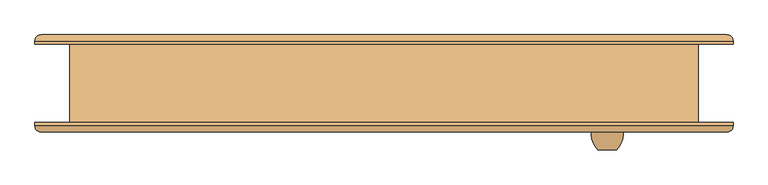
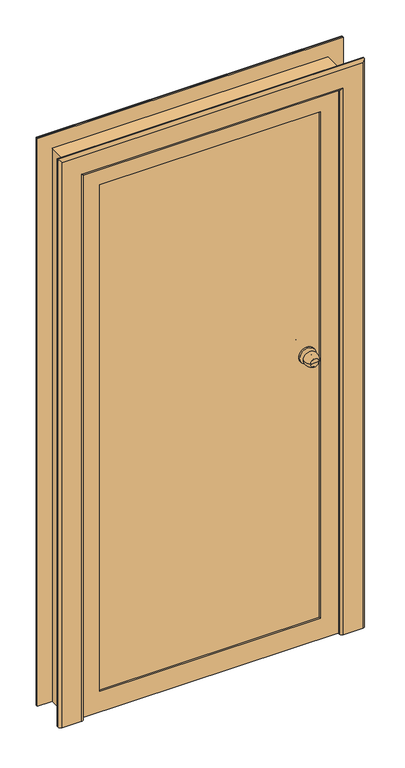
"""IFC4 building model written with IfcOpenShell, lengths in millimetres: door geometry, Наружная дверь 1-Навесная - Один проем наружу с порогом - 31173-2003 : ДСН КЛН  М1 УЗ 2100-1000 ГОСТ 31173-2003 2."""

from ifc_helpers import new_model, si_unit, point, frame, origin, place, context, project, spatial, polyline, circle_curve, ellipse_curve, trimmed, outline, extrude, faceted_brep, source, transform, mapped, element, save
from ifc_brep_helpers import plane_surface, cylinder_surface, revolved_surface, advanced_brep


def door_ae19c2ee(model_context):
    return source(origin(), model_context, "Body", "SolidModel", [
        advanced_brep(
        [(340.0, -105.5, 1100.0), (355.0, -105.5, 1100.0), (370.0, -105.5, 1100.0), (380.0, -75.5, 1100.0), (330.0, -75.5, 1100.0), (373.0, -75.5, 1100.0), (337.0, -75.5, 1100.0), (365.0, -67.5, 1100.0), (345.0, -67.5, 1100.0), (365.0, -61.5, 1100.0), (345.0, -61.5, 1100.0), (385.0, -61.5, 1100.0), (325.0, -61.5, 1100.0), (385.0, -55.5, 1100.0), (325.0, -55.5, 1100.0)],
        [
            (0, 1),
            (1, 2),
            (2, 0, circle_curve(frame((355.0, -105.5, 1100.0), z_axis=(0.0, -1.0, 0.0), x_axis=(1.0, 0.0, 0.0)), 15.0)),
            (0, 2, circle_curve(frame((355.0, -105.5, 1100.0), z_axis=(0.0, -1.0, 0.0), x_axis=(1.0, 0.0, 0.0)), 15.0)),
            (2, 3, circle_curve(frame((345.3773735, -80.6257912, 1100.0), z_axis=(0.0, 0.0, 1.0), x_axis=(-1.0, 0.0, 0.0)), 35.0)),
            (3, 4, circle_curve(frame((355.0, -75.5, 1100.0), z_axis=(0.0, -1.0, 0.0), x_axis=(1.0, 0.0, 0.0)), 25.0)),
            (4, 0, circle_curve(frame((364.6226265, -80.6257912, 1100.0), z_axis=(0.0, 0.0, 1.0), x_axis=(1.0, 0.0, 0.0)), 35.0)),
            (4, 3, circle_curve(frame((355.0, -75.5, 1100.0), z_axis=(0.0, -1.0, 0.0), x_axis=(1.0, 0.0, 0.0)), 25.0)),
            (3, 5),
            (5, 6, circle_curve(frame((355.0, -75.5, 1100.0), z_axis=(0.0, -1.0, 0.0), x_axis=(1.0, 0.0, 0.0)), 18.0)),
            (6, 4),
            (6, 5, circle_curve(frame((355.0, -75.5, 1100.0), z_axis=(0.0, -1.0, 0.0), x_axis=(1.0, 0.0, 0.0)), 18.0)),
            (5, 7, circle_curve(frame((373.0, -67.5, 1100.0), z_axis=(0.0, 0.0, -1.0), x_axis=(-1.0, 0.0, 0.0)), 8.0)),
            (7, 8, circle_curve(frame((355.0, -67.5, 1100.0), z_axis=(0.0, -1.0, 0.0), x_axis=(1.0, 0.0, 0.0)), 10.0)),
            (8, 6, circle_curve(frame((337.0, -67.5, 1100.0), z_axis=(0.0, 0.0, -1.0), x_axis=(1.0, 0.0, 0.0)), 8.0)),
            (8, 7, circle_curve(frame((355.0, -67.5, 1100.0), z_axis=(0.0, -1.0, 0.0), x_axis=(1.0, 0.0, 0.0)), 10.0)),
            (7, 9),
            (9, 10, circle_curve(frame((355.0, -61.5, 1100.0), z_axis=(0.0, -1.0, 0.0), x_axis=(1.0, 0.0, 0.0)), 10.0)),
            (10, 8),
            (10, 9, circle_curve(frame((355.0, -61.5, 1100.0), z_axis=(0.0, -1.0, 0.0), x_axis=(1.0, 0.0, 0.0)), 10.0)),
            (11, 12, circle_curve(frame((355.0, -61.5, 1100.0), z_axis=(0.0, -1.0, 0.0), x_axis=(-1.0, 0.0, 0.0)), 30.0)),
            (12, 11, circle_curve(frame((355.0, -61.5, 1100.0), z_axis=(0.0, -1.0, 0.0), x_axis=(-1.0, 0.0, 0.0)), 30.0)),
            (13, 14, circle_curve(frame((355.0, -55.5, 1100.0), z_axis=(0.0, 1.0, 0.0), x_axis=(-1.0, 0.0, 0.0)), 30.0)),
            (14, 13, circle_curve(frame((355.0, -55.5, 1100.0), z_axis=(0.0, 1.0, 0.0), x_axis=(-1.0, 0.0, 0.0)), 30.0)),
            (12, 14),
            (13, 11),
        ],
        [
            plane_surface(frame((355.0, -105.5, 1100.0), z_axis=(0.0, -1.0, 0.0), x_axis=(1.0, 0.0, 0.0))),
            revolved_surface(trimmed(ellipse_curve(frame((345.3773735, -80.6257912, 1100.0), z_axis=(0.0, 0.0, 1.0), x_axis=(-1.0, 0.0, 0.0)), 35.0, 35.0), [point((370.0, -105.5, 1100.0))], [point((380.0, -75.5, 1100.0))], True, "CARTESIAN"), (355.0, -135.5, 1100.0), (0.0, 1.0, 0.0)),
            plane_surface(frame((355.0, -75.5, 1100.0), z_axis=(0.0, 1.0, 0.0), x_axis=(1.0, 0.0, 0.0))),
            revolved_surface(trimmed(ellipse_curve(frame((373.0, -67.5, 1100.0), z_axis=(0.0, 0.0, -1.0), x_axis=(-1.0, 0.0, 0.0)), 8.0, 8.0), [point((373.0, -75.5, 1100.0))], [point((365.0, -67.5, 1100.0))], True, "CARTESIAN"), (355.0, -135.5, 1100.0), (0.0, 1.0, 0.0)),
            cylinder_surface(frame((355.0, -135.5, 1100.0), z_axis=(0.0, 1.0, 0.0), x_axis=(1.0, 0.0, 0.0)), 10.0),
            plane_surface(frame((325.0, -61.5, 1100.0), z_axis=(0.0, -1.0, 0.0), x_axis=(0.0, 0.0, 1.0))),
            plane_surface(frame((325.0, -55.5, 1100.0), z_axis=(0.0, 1.0, 0.0), x_axis=(0.0, 0.0, -1.0))),
            cylinder_surface(frame((355.0, -55.5, 1100.0), z_axis=(0.0, -1.0, 0.0), x_axis=(-1.0, 0.0, 0.0)), 30.0),
        ],
        [
            (0, [[1, 2, 3]]),
            (0, [[-1, 4, -2]]),
            (1, [[5, 6, 7, -3]]),
            (1, [[-7, 8, -5, -4]]),
            (2, [[9, 10, 11, -6]]),
            (2, [[-11, 12, -9, -8]]),
            (3, [[13, 14, 15, -10]]),
            (3, [[-15, 16, -13, -12]]),
            (4, [[17, 18, 19, -14]]),
            (4, [[-19, 20, -17, -16]]),
            (5, [[21, 22], [-20, -18]]),
            (6, [[23, 24]]),
            (7, [[25, -23, 26, -22]]),
            (7, [[-26, -24, -25, -21]]),
        ],
    ),
        advanced_brep(
        [(370.0, 64.5, 1100.0), (355.0, 64.5, 1100.0), (340.0, 64.5, 1100.0), (330.0, 34.5, 1100.0), (380.0, 34.5, 1100.0), (337.0, 34.5, 1100.0), (373.0, 34.5, 1100.0), (345.0, 26.5, 1100.0), (365.0, 26.5, 1100.0), (345.0, 20.5, 1100.0), (365.0, 20.5, 1100.0), (325.0, 20.5, 1100.0), (385.0, 20.5, 1100.0), (325.0, 14.5, 1100.0), (385.0, 14.5, 1100.0)],
        [
            (0, 1),
            (1, 2),
            (2, 0, circle_curve(frame((355.0, 64.5, 1100.0), z_axis=(0.0, 1.0, 0.0), x_axis=(-1.0, 0.0, 0.0)), 15.0)),
            (0, 2, circle_curve(frame((355.0, 64.5, 1100.0), z_axis=(0.0, 1.0, 0.0), x_axis=(-1.0, 0.0, 0.0)), 15.0)),
            (2, 3, circle_curve(frame((364.6226265, 39.6257912, 1100.0), z_axis=(0.0, 0.0, 1.0), x_axis=(1.0, 0.0, 0.0)), 35.0)),
            (3, 4, circle_curve(frame((355.0, 34.5, 1100.0), z_axis=(0.0, 1.0, 0.0), x_axis=(-1.0, 0.0, 0.0)), 25.0)),
            (4, 0, circle_curve(frame((345.3773735, 39.6257912, 1100.0), z_axis=(0.0, 0.0, 1.0), x_axis=(-1.0, 0.0, 0.0)), 35.0)),
            (4, 3, circle_curve(frame((355.0, 34.5, 1100.0), z_axis=(0.0, 1.0, 0.0), x_axis=(-1.0, 0.0, 0.0)), 25.0)),
            (3, 5),
            (5, 6, circle_curve(frame((355.0, 34.5, 1100.0), z_axis=(0.0, 1.0, 0.0), x_axis=(-1.0, 0.0, 0.0)), 18.0)),
            (6, 4),
            (6, 5, circle_curve(frame((355.0, 34.5, 1100.0), z_axis=(0.0, 1.0, 0.0), x_axis=(-1.0, 0.0, 0.0)), 18.0)),
            (5, 7, circle_curve(frame((337.0, 26.5, 1100.0), z_axis=(0.0, 0.0, -1.0), x_axis=(1.0, 0.0, 0.0)), 8.0)),
            (7, 8, circle_curve(frame((355.0, 26.5, 1100.0), z_axis=(0.0, 1.0, 0.0), x_axis=(-1.0, 0.0, 0.0)), 10.0)),
            (8, 6, circle_curve(frame((373.0, 26.5, 1100.0), z_axis=(0.0, 0.0, -1.0), x_axis=(-1.0, 0.0, 0.0)), 8.0)),
            (8, 7, circle_curve(frame((355.0, 26.5, 1100.0), z_axis=(0.0, 1.0, 0.0), x_axis=(-1.0, 0.0, 0.0)), 10.0)),
            (7, 9),
            (9, 10, circle_curve(frame((355.0, 20.5, 1100.0), z_axis=(0.0, 1.0, 0.0), x_axis=(-1.0, 0.0, 0.0)), 10.0)),
            (10, 8),
            (10, 9, circle_curve(frame((355.0, 20.5, 1100.0), z_axis=(0.0, 1.0, 0.0), x_axis=(-1.0, 0.0, 0.0)), 10.0)),
            (11, 12, circle_curve(frame((355.0, 20.5, 1100.0), z_axis=(0.0, 1.0, 0.0), x_axis=(1.0, 0.0, 0.0)), 30.0)),
            (12, 11, circle_curve(frame((355.0, 20.5, 1100.0), z_axis=(0.0, 1.0, 0.0), x_axis=(1.0, 0.0, 0.0)), 30.0)),
            (13, 14, circle_curve(frame((355.0, 14.5, 1100.0), z_axis=(0.0, -1.0, 0.0), x_axis=(1.0, 0.0, 0.0)), 30.0)),
            (14, 13, circle_curve(frame((355.0, 14.5, 1100.0), z_axis=(0.0, -1.0, 0.0), x_axis=(1.0, 0.0, 0.0)), 30.0)),
            (12, 14),
            (13, 11),
        ],
        [
            plane_surface(frame((355.0, 64.5, 1100.0), z_axis=(0.0, 1.0, 0.0), x_axis=(-1.0, 0.0, 0.0))),
            revolved_surface(trimmed(ellipse_curve(frame((364.6226265, 39.6257912, 1100.0), z_axis=(0.0, 0.0, 1.0), x_axis=(1.0, 0.0, 0.0)), 35.0, 35.0), [point((340.0, 64.5, 1100.0))], [point((330.0, 34.5, 1100.0))], True, "CARTESIAN"), (355.0, 94.5, 1100.0), (0.0, -1.0, 0.0)),
            plane_surface(frame((355.0, 34.5, 1100.0), z_axis=(0.0, -1.0, 0.0), x_axis=(-1.0, 0.0, 0.0))),
            revolved_surface(trimmed(ellipse_curve(frame((337.0, 26.5, 1100.0), z_axis=(0.0, 0.0, -1.0), x_axis=(1.0, 0.0, 0.0)), 8.0, 8.0), [point((337.0, 34.5, 1100.0))], [point((345.0, 26.5, 1100.0))], True, "CARTESIAN"), (355.0, 94.5, 1100.0), (0.0, -1.0, 0.0)),
            cylinder_surface(frame((355.0, 94.5, 1100.0), z_axis=(0.0, -1.0, 0.0), x_axis=(-1.0, 0.0, 0.0)), 10.0),
            plane_surface(frame((385.0, 20.5, 1100.0), z_axis=(0.0, 1.0, 0.0), x_axis=(0.0, 0.0, 1.0))),
            plane_surface(frame((385.0, 14.5, 1100.0), z_axis=(0.0, -1.0, 0.0), x_axis=(0.0, 0.0, -1.0))),
            cylinder_surface(frame((355.0, 14.5, 1100.0), z_axis=(0.0, 1.0, 0.0), x_axis=(1.0, 0.0, 0.0)), 30.0),
        ],
        [
            (0, [[1, 2, 3]]),
            (0, [[-1, 4, -2]]),
            (1, [[5, 6, 7, -3]]),
            (1, [[-7, 8, -5, -4]]),
            (2, [[9, 10, 11, -6]]),
            (2, [[-11, 12, -9, -8]]),
            (3, [[13, 14, 15, -10]]),
            (3, [[-15, 16, -13, -12]]),
            (4, [[17, 18, 19, -14]]),
            (4, [[-19, 20, -17, -16]]),
            (5, [[21, 22], [-20, -18]]),
            (6, [[23, 24]]),
            (7, [[25, -23, 26, -22]]),
            (7, [[-26, -24, -25, -21]]),
        ],
    ),
        faceted_brep([(435.0, 14.5, 42.0), (435.0, 9.5, 42.0), (-435.0, 9.5, 42.0), (-435.0, 14.5, 42.0), (435.0, 14.5, 2055.0), (435.0, 9.5, 2055.0), (-435.0, 9.5, 2055.0), (415.0, 9.5, 2035.0), (415.0, 9.5, 62.0), (-415.0, 9.5, 62.0), (-415.0, 9.5, 2035.0), (-435.0, 14.5, 2055.0), (415.0, -55.5, 2035.0), (415.0, -55.5, 62.0), (-415.0, -55.5, 62.0), (-415.0, -55.5, 2035.0)], [[[0, 1, 2, 3]], [[4, 5, 1, 0]], [[5, 6, 2, 1], [7, 8, 9, 10]], [[2, 6, 11, 3]], [[11, 4, 0, 3]], [[7, 12, 13, 8]], [[9, 8, 13, 14]], [[15, 10, 9, 14]], [[12, 15, 14, 13]], [[4, 11, 6, 5]], [[7, 10, 15, 12]]]),
        extrude(outline(polyline([(0.0, 465.0), (0.0, 480.0), (2100.0, 480.0), (2100.0, -480.0), (0.0, -480.0), (0.0, -465.0), (2085.0, -465.0), (2085.0, 465.0), (0.0, 465.0)])), frame((0.0, 7.5, 0.0), z_axis=(0.0, 1.0, 0.0), x_axis=(0.0, 0.0, 1.0)), (0.0, 0.0, 1.0), 55.0),
        faceted_brep([(480.0, 7.5, 0.0), (480.0, -62.5, 0.0), (-480.0, -62.5, 0.0), (-480.0, 7.5, 0.0), (-480.0, -62.5, 2100.0), (-480.0, 7.5, 2100.0), (480.0, -62.5, 2100.0), (-400.0, -62.5, 2020.0), (400.0, -62.5, 2020.0), (400.0, -62.5, 80.0), (-400.0, -62.5, 80.0), (480.0, 7.5, 2100.0), (-420.0, 7.5, 60.0), (420.0, 7.5, 60.0), (420.0, 7.5, 2040.0), (-420.0, 7.5, 2040.0), (420.0, -57.5, 60.0), (-420.0, -57.5, 60.0), (-420.0, -57.5, 2040.0), (420.0, -57.5, 2040.0), (-400.0, -57.5, 80.0), (400.0, -57.5, 80.0), (400.0, -57.5, 2020.0), (-400.0, -57.5, 2020.0)], [[[0, 1, 2, 3]], [[3, 2, 4, 5]], [[2, 1, 6, 4], [7, 8, 9, 10]], [[5, 11, 0, 3], [12, 13, 14, 15]], [[16, 13, 12, 17]], [[17, 12, 15, 18]], [[18, 19, 16, 17], [20, 21, 22, 23]], [[9, 21, 20, 10]], [[10, 20, 23, 7]], [[11, 6, 1, 0]], [[19, 14, 13, 16]], [[8, 22, 21, 9]], [[5, 4, 6, 11]], [[18, 15, 14, 19]], [[7, 23, 22, 8]]]),
        advanced_brep(
        [(-555.0, -62.5, 0.0), (-465.0, -62.5, 0.0), (-465.0, -67.5, 0.0), (-475.0, -77.5, 0.0), (-545.0, -77.5, 0.0), (-555.0, -67.5, 0.0), (-555.0, -62.5, 2175.0), (555.0, -62.5, 2175.0), (555.0, -62.5, 0.0), (465.0, -62.5, 0.0), (465.0, -62.5, 2085.0), (-465.0, -62.5, 2085.0), (-465.0, -67.5, 2085.0), (-475.0, -77.5, 2095.0), (475.0, -77.5, 2095.0), (475.0, -77.5, 0.0), (545.0, -77.5, 0.0), (545.0, -77.5, 2165.0), (-545.0, -77.5, 2165.0), (-555.0, -67.5, 2175.0), (555.0, -67.5, 2175.0), (555.0, -67.5, 0.0), (465.0, -67.5, 0.0), (465.0, -67.5, 2085.0)],
        [
            (0, 1),
            (1, 2),
            (2, 3, circle_curve(frame((-475.0, -67.5, 0.0), z_axis=(0.0, 0.0, -1.0), x_axis=(-1.0, 0.0, 0.0)), 10.0)),
            (3, 4),
            (4, 5, circle_curve(frame((-545.0, -67.5, 0.0), z_axis=(0.0, 0.0, -1.0), x_axis=(-1.0, 0.0, 0.0)), 10.0)),
            (5, 0),
            (0, 6),
            (6, 7),
            (7, 8),
            (8, 9),
            (9, 10),
            (10, 11),
            (11, 1),
            (11, 12),
            (12, 2),
            (12, 13, ellipse_curve(frame((-475.0, -67.5, 2095.0), z_axis=(-0.7071067811865475, 0.0, -0.7071067811865475), x_axis=(0.7071067811865474, 0.0, -0.7071067811865476)), 14.1421356, 10.0)),
            (13, 3),
            (13, 14),
            (14, 15),
            (15, 16),
            (16, 17),
            (17, 18),
            (18, 4),
            (18, 19, ellipse_curve(frame((-545.0, -67.5, 2165.0), z_axis=(-0.7071067811865475, 0.0, -0.7071067811865475), x_axis=(0.7071067811865474, 0.0, -0.7071067811865476)), 14.1421356, 10.0)),
            (19, 5),
            (19, 6),
            (7, 20),
            (20, 21),
            (21, 8),
            (21, 16, circle_curve(frame((545.0, -67.5, 0.0), z_axis=(0.0, 0.0, -1.0), x_axis=(1.0, 0.0, 0.0)), 10.0)),
            (15, 22, circle_curve(frame((475.0, -67.5, 0.0), z_axis=(0.0, 0.0, -1.0), x_axis=(1.0, 0.0, 0.0)), 10.0)),
            (22, 9),
            (23, 10),
            (22, 23),
            (14, 23, ellipse_curve(frame((475.0, -67.5, 2095.0), z_axis=(0.7071067811865475, 0.0, -0.7071067811865475), x_axis=(0.7071067811865474, 0.0, 0.7071067811865476)), 14.1421356, 10.0)),
            (20, 17, ellipse_curve(frame((545.0, -67.5, 2165.0), z_axis=(0.7071067811865475, 0.0, -0.7071067811865475), x_axis=(0.7071067811865474, 0.0, 0.7071067811865476)), 14.1421356, 10.0)),
            (23, 12),
            (20, 19),
        ],
        [
            plane_surface(frame((-500.0, -62.5, 0.0), z_axis=(0.0, 0.0, -1.0), x_axis=(0.0, -1.0, 0.0))),
            plane_surface(frame((-555.0, -62.5, 0.0), z_axis=(0.0, 1.0, 0.0), x_axis=(0.0, 0.0, 1.0))),
            plane_surface(frame((-465.0, -62.5, 0.0), z_axis=(1.0, 0.0, 0.0), x_axis=(0.0, 0.0, 1.0))),
            cylinder_surface(frame((-475.0, -67.5, 0.0), z_axis=(0.0, 0.0, -1.0), x_axis=(-1.0, 0.0, 0.0)), 10.0),
            plane_surface(frame((-475.0, -77.5, 0.0), z_axis=(0.0, -1.0, 0.0), x_axis=(0.0, 0.0, 1.0))),
            cylinder_surface(frame((-545.0, -67.5, 0.0), z_axis=(0.0, 0.0, -1.0), x_axis=(-1.0, 0.0, 0.0)), 10.0),
            plane_surface(frame((-555.0, -67.5, 0.0), z_axis=(-1.0, 0.0, 0.0), x_axis=(0.0, 0.0, 1.0))),
            plane_surface(frame((555.0, -67.5, 2175.0), z_axis=(1.0, 0.0, 0.0), x_axis=(0.0, 0.0, -1.0))),
            plane_surface(frame((500.0, -62.5, 0.0), z_axis=(0.0, 0.0, -1.0), x_axis=(0.0, -1.0, 0.0))),
            plane_surface(frame((465.0, -62.5, 2085.0), z_axis=(-1.0, 0.0, 0.0), x_axis=(0.0, 0.0, -1.0))),
            cylinder_surface(frame((475.0, -67.5, 2120.0), z_axis=(0.0, 0.0, 1.0), x_axis=(1.0, 0.0, 0.0)), 10.0),
            cylinder_surface(frame((545.0, -67.5, 2120.0), z_axis=(0.0, 0.0, 1.0), x_axis=(1.0, 0.0, 0.0)), 10.0),
            plane_surface(frame((-465.0, -62.5, 2085.0), z_axis=(0.0, 0.0, -1.0), x_axis=(1.0, 0.0, 0.0))),
            cylinder_surface(frame((-500.0, -67.5, 2095.0), z_axis=(-1.0, 0.0, 0.0), x_axis=(0.0, 0.0, 1.0)), 10.0),
            cylinder_surface(frame((-500.0, -67.5, 2165.0), z_axis=(-1.0, 0.0, 0.0), x_axis=(0.0, 0.0, 1.0)), 10.0),
            plane_surface(frame((-555.0, -67.5, 2175.0), z_axis=(0.0, 0.0, 1.0), x_axis=(1.0, 0.0, 0.0))),
        ],
        [
            (0, [[1, 2, 3, 4, 5, 6]]),
            (1, [[-1, 7, 8, 9, 10, 11, 12, 13]]),
            (2, [[-2, -13, 14, 15]]),
            (3, [[-3, -15, 16, 17]]),
            (4, [[-4, -17, 18, 19, 20, 21, 22, 23]]),
            (5, [[-5, -23, 24, 25]]),
            (6, [[-6, -25, 26, -7]]),
            (7, [[27, 28, 29, -9]]),
            (8, [[-29, 30, -20, 31, 32, -10]]),
            (9, [[33, -11, -32, 34]]),
            (10, [[35, -34, -31, -19]]),
            (11, [[36, -21, -30, -28]]),
            (12, [[-14, -12, -33, 37]]),
            (13, [[-16, -37, -35, -18]]),
            (14, [[-24, -22, -36, 38]]),
            (15, [[-26, -38, -27, -8]]),
        ],
    ),
        advanced_brep(
        [(555.0, 62.5, 0.0), (465.0, 62.5, 0.0), (465.0, 67.5, 0.0), (475.0, 77.5, 0.0), (545.0, 77.5, 0.0), (555.0, 67.5, 0.0), (555.0, 62.5, 2175.0), (-555.0, 62.5, 2175.0), (-555.0, 62.5, 0.0), (-465.0, 62.5, 0.0), (-465.0, 62.5, 2085.0), (465.0, 62.5, 2085.0), (465.0, 67.5, 2085.0), (475.0, 77.5, 2095.0), (-475.0, 77.5, 2095.0), (-475.0, 77.5, 0.0), (-545.0, 77.5, 0.0), (-545.0, 77.5, 2165.0), (545.0, 77.5, 2165.0), (555.0, 67.5, 2175.0), (-555.0, 67.5, 2175.0), (-555.0, 67.5, 0.0), (-465.0, 67.5, 0.0), (-465.0, 67.5, 2085.0)],
        [
            (0, 1),
            (1, 2),
            (2, 3, circle_curve(frame((475.0, 67.5, 0.0), z_axis=(0.0, 0.0, -1.0), x_axis=(1.0, 0.0, 0.0)), 10.0)),
            (3, 4),
            (4, 5, circle_curve(frame((545.0, 67.5, 0.0), z_axis=(0.0, 0.0, -1.0), x_axis=(1.0, 0.0, 0.0)), 10.0)),
            (5, 0),
            (0, 6),
            (6, 7),
            (7, 8),
            (8, 9),
            (9, 10),
            (10, 11),
            (11, 1),
            (11, 12),
            (12, 2),
            (12, 13, ellipse_curve(frame((475.0, 67.5, 2095.0), z_axis=(0.7071067811865475, 0.0, -0.7071067811865475), x_axis=(-0.7071067811865474, 0.0, -0.7071067811865476)), 14.1421356, 10.0)),
            (13, 3),
            (13, 14),
            (14, 15),
            (15, 16),
            (16, 17),
            (17, 18),
            (18, 4),
            (18, 19, ellipse_curve(frame((545.0, 67.5, 2165.0), z_axis=(0.7071067811865475, 0.0, -0.7071067811865475), x_axis=(-0.7071067811865474, 0.0, -0.7071067811865476)), 14.1421356, 10.0)),
            (19, 5),
            (19, 6),
            (7, 20),
            (20, 21),
            (21, 8),
            (21, 16, circle_curve(frame((-545.0, 67.5, 0.0), z_axis=(0.0, 0.0, -1.0), x_axis=(-1.0, 0.0, 0.0)), 10.0)),
            (15, 22, circle_curve(frame((-475.0, 67.5, 0.0), z_axis=(0.0, 0.0, -1.0), x_axis=(-1.0, 0.0, 0.0)), 10.0)),
            (22, 9),
            (23, 10),
            (22, 23),
            (14, 23, ellipse_curve(frame((-475.0, 67.5, 2095.0), z_axis=(-0.7071067811865475, 0.0, -0.7071067811865475), x_axis=(-0.7071067811865474, 0.0, 0.7071067811865476)), 14.1421356, 10.0)),
            (20, 17, ellipse_curve(frame((-545.0, 67.5, 2165.0), z_axis=(-0.7071067811865475, 0.0, -0.7071067811865475), x_axis=(-0.7071067811865474, 0.0, 0.7071067811865476)), 14.1421356, 10.0)),
            (23, 12),
            (20, 19),
        ],
        [
            plane_surface(frame((500.0, 62.5, 0.0), z_axis=(0.0, 0.0, -1.0), x_axis=(0.0, -1.0, 0.0))),
            plane_surface(frame((555.0, 62.5, 0.0), z_axis=(0.0, -1.0, 0.0), x_axis=(0.0, 0.0, 1.0))),
            plane_surface(frame((465.0, 62.5, 0.0), z_axis=(-1.0, 0.0, 0.0), x_axis=(0.0, 0.0, 1.0))),
            cylinder_surface(frame((475.0, 67.5, 0.0), z_axis=(0.0, 0.0, -1.0), x_axis=(1.0, 0.0, 0.0)), 10.0),
            plane_surface(frame((475.0, 77.5, 0.0), z_axis=(0.0, 1.0, 0.0), x_axis=(0.0, 0.0, 1.0))),
            cylinder_surface(frame((545.0, 67.5, 0.0), z_axis=(0.0, 0.0, -1.0), x_axis=(1.0, 0.0, 0.0)), 10.0),
            plane_surface(frame((555.0, 67.5, 0.0), z_axis=(1.0, 0.0, 0.0), x_axis=(0.0, 0.0, 1.0))),
            plane_surface(frame((-555.0, 67.5, 2175.0), z_axis=(-1.0, 0.0, 0.0), x_axis=(0.0, 0.0, -1.0))),
            plane_surface(frame((-500.0, 62.5, 0.0), z_axis=(0.0, 0.0, -1.0), x_axis=(0.0, -1.0, 0.0))),
            plane_surface(frame((-465.0, 62.5, 2085.0), z_axis=(1.0, 0.0, 0.0), x_axis=(0.0, 0.0, -1.0))),
            cylinder_surface(frame((-475.0, 67.5, 2120.0), z_axis=(0.0, 0.0, 1.0), x_axis=(-1.0, 0.0, 0.0)), 10.0),
            cylinder_surface(frame((-545.0, 67.5, 2120.0), z_axis=(0.0, 0.0, 1.0), x_axis=(-1.0, 0.0, 0.0)), 10.0),
            plane_surface(frame((465.0, 62.5, 2085.0), z_axis=(0.0, 0.0, -1.0), x_axis=(-1.0, 0.0, 0.0))),
            cylinder_surface(frame((500.0, 67.5, 2095.0), z_axis=(1.0, 0.0, 0.0), x_axis=(0.0, 0.0, 1.0)), 10.0),
            cylinder_surface(frame((500.0, 67.5, 2165.0), z_axis=(1.0, 0.0, 0.0), x_axis=(0.0, 0.0, 1.0)), 10.0),
            plane_surface(frame((555.0, 67.5, 2175.0), z_axis=(0.0, 0.0, 1.0), x_axis=(-1.0, 0.0, 0.0))),
        ],
        [
            (0, [[1, 2, 3, 4, 5, 6]]),
            (1, [[-1, 7, 8, 9, 10, 11, 12, 13]]),
            (2, [[-2, -13, 14, 15]]),
            (3, [[-3, -15, 16, 17]]),
            (4, [[-4, -17, 18, 19, 20, 21, 22, 23]]),
            (5, [[-5, -23, 24, 25]]),
            (6, [[-6, -25, 26, -7]]),
            (7, [[27, 28, 29, -9]]),
            (8, [[-29, 30, -20, 31, 32, -10]]),
            (9, [[33, -11, -32, 34]]),
            (10, [[35, -34, -31, -19]]),
            (11, [[36, -21, -30, -28]]),
            (12, [[-14, -12, -33, 37]]),
            (13, [[-16, -37, -35, -18]]),
            (14, [[-24, -22, -36, 38]]),
            (15, [[-26, -38, -27, -8]]),
        ],
    ),
        extrude(outline(polyline([(0.0, 480.0), (0.0, 500.0), (2120.0, 500.0), (2120.0, -500.0), (0.0, -500.0), (0.0, -480.0), (2100.0, -480.0), (2100.0, 480.0), (0.0, 480.0)])), frame((0.0, -62.5, 0.0), z_axis=(0.0, 1.0, 0.0), x_axis=(0.0, 0.0, 1.0)), (0.0, 0.0, 1.0), 125.0),
    ])


if __name__ == "__main__":
    model = new_model("IFC4")
    model_context = context("Model", 3, world=origin())
    ifc_project = project(units=[si_unit("LENGTHUNIT", "METRE", prefix="MILLI")], contexts=[model_context])
    site = spatial("IfcSite", under=ifc_project)
    building = spatial("IfcBuilding", under=site)
    placement = place(None, origin())
    door_shape = door_ae19c2ee(model_context)
    element("IfcDoor", 1, ObjectType="Наружная дверь 1-Навесная - Один проем наружу с порогом - 31173-2003 : ДСН КЛН  М1 УЗ 2100-1000 ГОСТ 31173-2003 2", at=placement, inside=building, context=model_context, shape_type="MappedRepresentation", body=[
        mapped(door_shape, transform((0.0, 0.0, 0.0), x_axis=(1.0, 0.0, 0.0), y_axis=(0.0, 1.0, 0.0), z_axis=(0.0, 0.0, 1.0))),
    ])
    save(model, "model.ifc")

# Revit data of these elements
# Type "Наружная дверь 1-Навесная - Один проем наружу с порогом - 31173-2003 : ДСН КЛН  М1 УЗ 2100-1000 ГОСТ 31173-2003 2"
#   Type Mark = "149"
#   Description = "ДСН КЛН  М1 УЗ 2100-900 ГОСТ 31173-2003"
#   Проекционное соединение по ширине = 90 mm
#   Rough Width = 1000 mm
#   Rough Height = 2120 mm
#   Угол проема [instance default] = 30°
#   Толщина_Тепл_Изоляции = 20 mm
#   Heat Transfer Coefficient (U) = 3.7021 W/(m²·K)
#   Height = 2100 mm
#   Width = 960 mm
#   Ширина каркаса = 60 mm
#   Толщина каркаса = 70 mm
#   Вставка двери [instance default] = 0 mm
#   Правая сторона = no
#   Левая сторона = yes
#   Function = 1
#   Обрезка = Сталь
#   Панель = Сталь
#   Тепловая изоляция = Тепловая изоляция
#   Кадр = Сталь
#   Дверная ручка = Металл
#   Visual Light Transmittance = 0
#   Solar Heat Gain Coefficient = 0
#   Construction Type Id = ""
#   Wall Closure = (empty or 0)
#   Analytic Construction = (empty or 0)
# Element 1 (IfcDoor, "Наружная дверь 1-Навесная - Один проем наружу с порогом - 31173-2003 : ДСН КЛН  М1 УЗ 2100-1000 ГОСТ 31173-2003 2")
#   Materials on its faces: "Сталь", "Металл", "Тепловая изоляция"
# Materials
#   "Сталь": class "Металл", colour RGB 247 247 247, transparency 0
#   "Тепловая изоляция": class "Пластмасса", colour RGB 185 154 119, transparency 0, Cost = 0
#   "Металл": class "Металл", colour RGB 249 249 249, transparency 0
